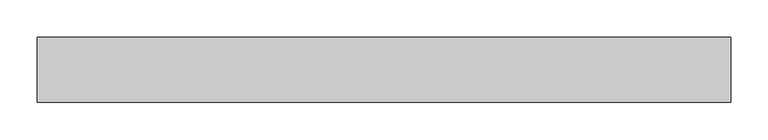
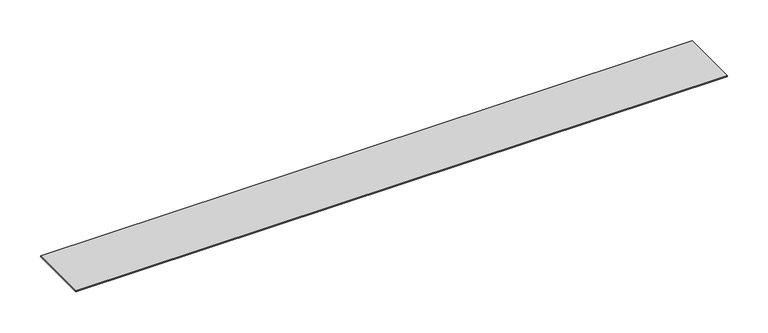
"""IFC4 building model written with IfcOpenShell, lengths in millimetres: proxy geometry, Generic Models 6:Generic Models 2:318829:Generic Models 2:318829 : Generic Models 6:Generic Models 2:318829:6 : Generic Models 6:Generic Models 2:318829:Generic Models 2:318829 : Generic Models 6:Generic Models 2:318829:300683."""

from ifc_helpers import new_model, si_unit, frame, origin, place, context, project, spatial, polyline, outline, extrude, source, transform, mapped, element, save


def generic_models_1178c1a7(model_context):
    return source(origin(), model_context, "Body", "SweptSolid", [
        extrude(outline(polyline([(570394.5036635, -579002.9006209), (570394.5036635, -579089.5913841), (569469.9742239, -579089.5913841), (569469.9742239, -579002.9006209), (570394.5036635, -579002.9006209)])), frame((0.0, 0.0, 25.3598442), z_axis=(0.0, 0.0, 1.0), x_axis=(1.0, 0.0, 0.0)), (0.0, 0.0, 1.0), 1.4049011),
    ])


if __name__ == "__main__":
    model = new_model("IFC4")
    model_context = context("Model", 3, world=origin())
    ifc_project = project(units=[si_unit("LENGTHUNIT", "METRE", prefix="MILLI")], contexts=[model_context])
    site = spatial("IfcSite", under=ifc_project)
    building = spatial("IfcBuilding", under=site)
    placement = place(None, origin())
    generic_models_shape = generic_models_1178c1a7(model_context)
    element("IfcBuildingElementProxy", 1, Name="Generic Models 6:Generic Models 2:318829:Generic Models 2:318829 : Generic Models 6:Generic Models 2:318829:6 : Generic Models 6:Generic Models 2:318829:Generic Models 2:318829 : Generic Models 6:Generic Models 2:318829:300683", ObjectType="Generic Models 6:Generic Models 2:318829:Generic Models 2:318829 : Generic Models 6:Generic Models 2:318829:6 : Generic Models 6:Generic Models 2:318829:Generic Models 2:318829 : Generic Models 6:Generic Models 2:318829:300683", at=placement, inside=building, context=model_context, shape_type="MappedRepresentation", body=[
        mapped(generic_models_shape, transform((0.0, 0.0, 0.0), x_axis=(1.0, 0.0, 0.0), y_axis=(0.0, 1.0, 0.0), z_axis=(0.0, 0.0, 1.0))),
    ])
    save(model, "model.ifc")

# Revit data of these elements
# Type "Generic Models 6:Generic Models 2:318829:Generic Models 2:318829 : Generic Models 6:Generic Models 2:318829:6 : Generic Models 6:Generic Models 2:318829:Generic Models 2:318829 : Generic Models 6:Generic Models 2:318829:300683"
#   NameOverride = "Generic Models 6:Generic Models 2:318829:Generic Models 2:318829 : Generic Models 6:Generic Models 2:318829:300683"
#   ObjectTypeOverride = "Generic Models 2:318829 : Generic Models 6:Generic Models 2:318829"
#   Reference = "Generic Models 2"
#   Tag = "300683"
# Element 1 (IfcBuildingElementProxy, "Generic Models 6:Generic Models 2:318829:Generic Models 2:318829 : Generic Models 6:Generic Models 2:318829:6 : Generic Models 6:Generic Models 2:318829:Generic Models 2:318829 : Generic Models 6:Generic Models 2:318829:300683")
#   Materials on its faces: "COMPRESSIBE THERMAL GASKET SANDWICHED BETWEEN METAL COMPONENTS"
# Materials
#   "COMPRESSIBE THERMAL GASKET SANDWICHED BETWEEN METAL COMPONENTS": class "Unassigned", colour RGB 58 208 21, transparency 0, Cost = 0
